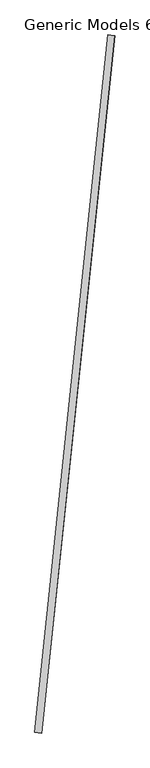
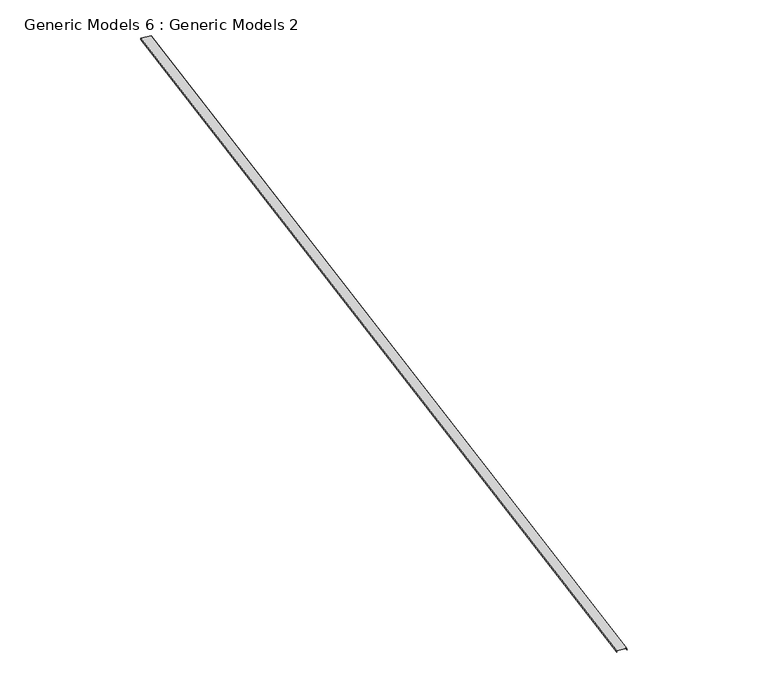
"""IFC4 building model written with IfcOpenShell, lengths in millimetres: proxy geometry, Generic Models 6 : Generic Models 2."""

from ifc_helpers import new_model, si_unit, frame, origin, place, context, project, spatial, polyline, outline, extrude, source, transform, mapped, element, save


def generic_models_6_generic_models_2_b984bb09(model_context):
    return source(origin(), model_context, "Body", "SweptSolid", [
        extrude(outline(polyline([(-1.5875, 0.0), (18.392436, 0.0), (22.417596, -4.02516), (21.295064, -5.1476921), (17.7348719, -1.5875), (-3.175, -1.5875), (-3.175, 134.9375), (22.225, 134.9375), (22.225, 133.3500001), (-1.5875, 133.3500001), (-1.5875, 0.0)])), frame((33803.3938485, 25673.8898408, 266407.9), z_axis=(0.10452846326765233, 0.9945218953682735, 0.0), x_axis=(1.7379143628849107e-12, 0.0, -1.0)), (0.0, 0.0, 1.0), 14138.3561194),
    ])


if __name__ == "__main__":
    model = new_model("IFC4")
    model_context = context("Model", 3, world=origin())
    ifc_project = project(units=[si_unit("LENGTHUNIT", "METRE", prefix="MILLI")], contexts=[model_context])
    site = spatial("IfcSite", under=ifc_project)
    building = spatial("IfcBuilding", under=site)
    placement = place(None, origin())
    generic_models_6_generic_models_2_shape = generic_models_6_generic_models_2_b984bb09(model_context)
    element("IfcBuildingElementProxy", 1, Name="Generic Models 6 : Generic Models 2", ObjectType="Generic Models 6 : Generic Models 2", at=placement, inside=building, context=model_context, shape_type="MappedRepresentation", body=[
        mapped(generic_models_6_generic_models_2_shape, transform((0.0, 0.0, 0.0), x_axis=(1.0, 0.0, 0.0), y_axis=(0.0, 1.0, 0.0), z_axis=(0.0, 0.0, 1.0))),
    ])
    save(model, "model.ifc")

# Revit data of these elements
# Element 1 (IfcBuildingElementProxy, "Generic Models 6 : Generic Models 2")
#   Materials on its faces: "GALV. BRAKE METAL - (COLOR: DARK BRONZE)"
# Materials
#   "GALV. BRAKE METAL - (COLOR: DARK BRONZE)": class "Generic", colour RGB 72 52 47, transparency 0, Cost = 0
